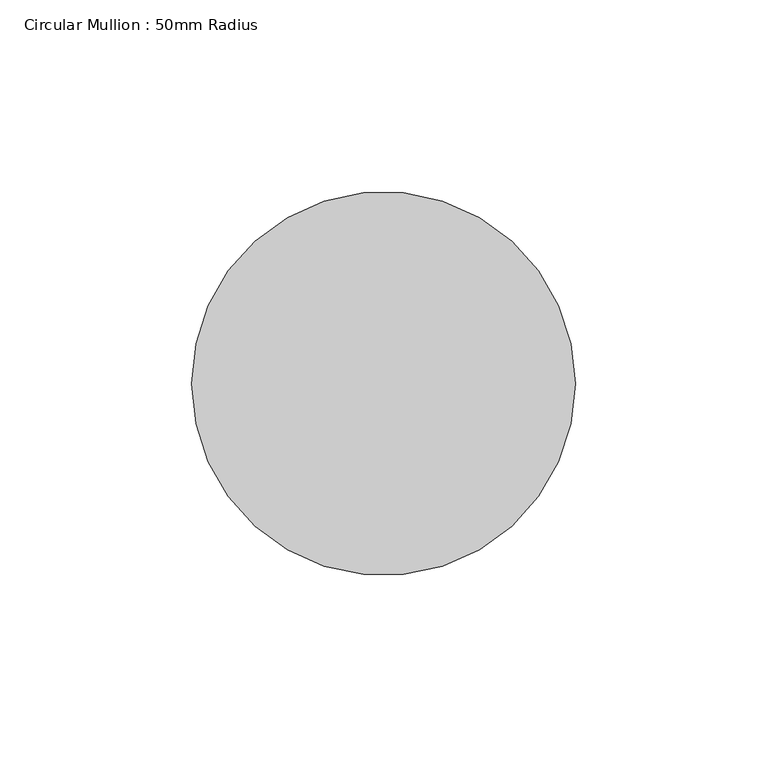
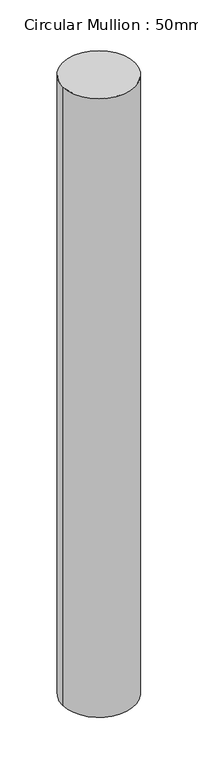
"""IFC4 building model written with IfcOpenShell, lengths in millimetres: member geometry, Circular Mullion : 50mm Radius."""

from ifc_helpers import new_model, si_unit, point, frame, origin, origin_2d, place, context, project, spatial, circle_curve, trimmed, segment, composite_curve, outline, extrude, source, transform, mapped, element, save


def circular_mullion_50mm_radius_a5acfd35(model_context):
    return source(origin(), model_context, "Body", "SweptSolid", [
        extrude(outline(composite_curve([segment(trimmed(circle_curve(origin_2d(), 50.0), [point((50.0, 0.0))], [point((-50.0, 0.0))], False, "CARTESIAN"), True, "CONTINUOUS"), segment(trimmed(circle_curve(origin_2d(), 50.0), [point((-50.0, 0.0))], [point((50.0, 0.0))], False, "CARTESIAN"), True, "CONTINUOUS")], self_intersect=False)), frame((0.0, 0.0, -902.1770932), z_axis=(0.0, 0.0, 1.0), x_axis=(1.0, 0.0, 0.0)), (0.0, 0.0, 1.0), 902.1770932),
    ])


if __name__ == "__main__":
    model = new_model("IFC4")
    model_context = context("Model", 3, world=origin())
    ifc_project = project(units=[si_unit("LENGTHUNIT", "METRE", prefix="MILLI")], contexts=[model_context])
    site = spatial("IfcSite", under=ifc_project)
    building = spatial("IfcBuilding", under=site)
    placement = place(None, origin())
    circular_mullion_50mm_radius_shape = circular_mullion_50mm_radius_a5acfd35(model_context)
    element("IfcMember", 1, ObjectType="Circular Mullion : 50mm Radius", at=placement, inside=building, context=model_context, shape_type="MappedRepresentation", body=[
        mapped(circular_mullion_50mm_radius_shape, transform((0.0, 0.0, 0.0), x_axis=(1.0, 0.0, 0.0), y_axis=(0.0, 1.0, 0.0), z_axis=(0.0, 0.0, 1.0))),
    ])
    save(model, "model.ifc")

# Revit data of these elements
# Type "Circular Mullion : 50mm Radius"
#   built-in parameter 1007350 = 0.164042 (stored number, unit not read)
# Element 1 (IfcMember, "Circular Mullion : 50mm Radius")
#   Materials on its faces: "Aluminium"
# Materials
#   "Aluminium": class "Metal", colour RGB 247 247 247, transparency 0, Description = "Aluminium 6061", Cost = 0
